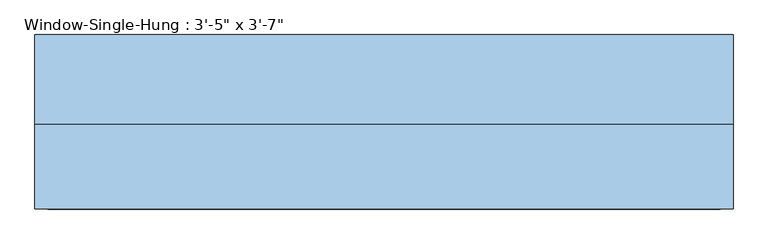
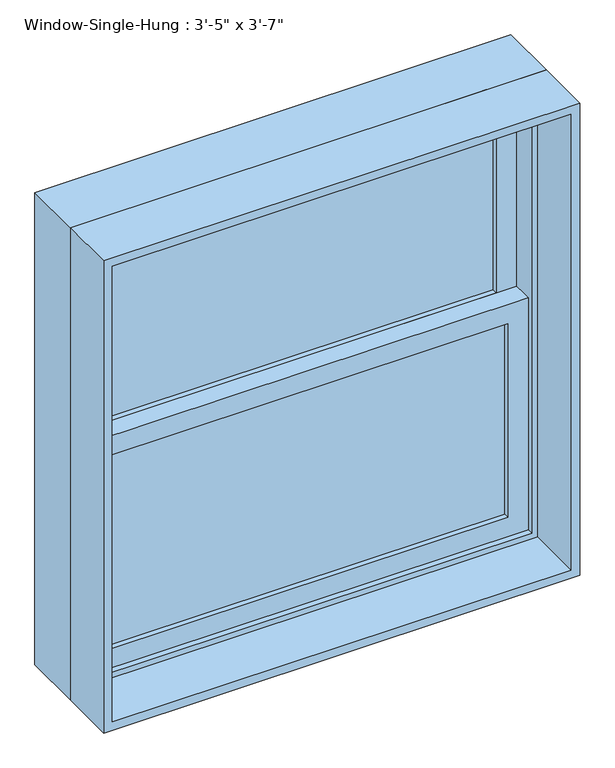
"""IFC4 building model written with IfcOpenShell, lengths in millimetres: window geometry."""

import ifcopenshell
import ifcopenshell.guid

model = None  # the IFC model being written
_history = None  # IfcOwnerHistory: only IFC2X3 demands one
_inside = {}  # id of a spatial element -> (the spatial element, [elements in it])
_under = {}  # id of a project, library or spatial element -> (it, [spatial elements below it])
_declared = {}  # id of a project -> (the project, [libraries it declares])
_typed = {}  # id of a type object -> (the type object, [elements of that type])
_made_of = {}  # id of a material, layer set ... -> (it, [elements and type objects made of it])


def new_model(schema):
    """Start an empty IFC model of exactly this schema.

    Asked for "IFC4X3", IfcOpenShell would pick the latest addendum, in which some entities
    have other attributes; the version numbers below select the first issue.
    IFC2X3 requires an IfcOwnerHistory on every rooted entity: one is made here for all.
    """
    global model, _history
    if schema == "IFC4X3":
        model = ifcopenshell.file(schema_version=(4, 3, 0, 0))
    else:
        model = ifcopenshell.file(schema=schema)
    _inside.clear()
    _under.clear()
    _declared.clear()
    _typed.clear()
    _made_of.clear()
    _history = None
    if model.schema == "IFC2X3":
        org = make("IfcOrganization", Name="unknown")
        user = make(
            "IfcPersonAndOrganization",
            ThePerson=make("IfcPerson", FamilyName="unknown"),
            TheOrganization=org,
        )
        app = make(
            "IfcApplication",
            ApplicationDeveloper=org,
            Version="unknown",
            ApplicationFullName="unknown",
            ApplicationIdentifier="unknown",
        )
        _history = make(
            "IfcOwnerHistory",
            OwningUser=user,
            OwningApplication=app,
            ChangeAction="ADDED",
            CreationDate=0,
        )
    return model


def make(cls, **values):
    """One entity of the class cls with the attributes given. An attribute that is None is left unset."""
    return model.create_entity(
        cls, **{name: value for name, value in values.items() if value is not None}
    )


def rooted(cls, **values):
    """An entity with a GlobalId (a new one), such as an element, a storey or a relation."""
    return make(cls, GlobalId=ifcopenshell.guid.new(), OwnerHistory=_history, **values)


def si_unit(unit_type, name, prefix=None):
    """IfcSIUnit, for example si_unit("LENGTHUNIT", "METRE", prefix="MILLI")."""
    return make("IfcSIUnit", UnitType=unit_type, Prefix=prefix, Name=name)


def assignment(units):
    """IfcUnitAssignment: the units of a project."""
    return None if units is None else make("IfcUnitAssignment", Units=units)


def point(xyz):
    """IfcCartesianPoint."""
    return None if xyz is None else make("IfcCartesianPoint", Coordinates=xyz)


def direction(xyz):
    """IfcDirection."""
    return None if xyz is None else make("IfcDirection", DirectionRatios=xyz)


def frame(location, z_axis=None, x_axis=None):
    """IfcAxis2Placement3D, a coordinate frame: its origin and axes. An axis left out is left unset."""
    return make(
        "IfcAxis2Placement3D",
        Location=point(location),
        Axis=direction(z_axis),
        RefDirection=direction(x_axis),
    )


def origin():
    """The frame at (0, 0, 0) with its axes left unset."""
    return frame((0.0, 0.0, 0.0))


def place(relative_to, where):
    """IfcLocalPlacement: puts the frame where relative to a parent placement (None: the world)."""
    return make(
        "IfcLocalPlacement", PlacementRelTo=relative_to, RelativePlacement=where
    )


def context(
    kind, dimensions, precision=None, world=None, true_north=None, identifier=None
):
    """IfcGeometricRepresentationContext, for example the 3D "Model" context."""
    return make(
        "IfcGeometricRepresentationContext",
        ContextIdentifier=identifier,
        ContextType=kind,
        CoordinateSpaceDimension=dimensions,
        Precision=precision,
        WorldCoordinateSystem=world,
        TrueNorth=true_north,
    )


def project(units=None, contexts=None):
    """IfcProject with its units and contexts."""
    return rooted(
        "IfcProject",
        Name="project",
        RepresentationContexts=contexts,
        UnitsInContext=assignment(units),
    )


def spatial(cls, under=None, at=None, **own):
    """A site, building, storey or space (cls), placed at a placement, below another one or the project."""
    s = rooted(cls, ObjectPlacement=at, **own)
    if under is not None:
        _under.setdefault(under.id(), (under, []))[1].append(s)
    return s


def polyline(points):
    """IfcPolyline through the points."""
    return make("IfcPolyline", Points=[point(p) for p in points])


def outline(outer, holes=None, kind="AREA"):
    """IfcArbitraryClosedProfileDef: a profile drawn as a closed curve; with holes, ...WithVoids."""
    if holes is None:
        return make("IfcArbitraryClosedProfileDef", ProfileType=kind, OuterCurve=outer)
    return make(
        "IfcArbitraryProfileDefWithVoids",
        ProfileType=kind,
        OuterCurve=outer,
        InnerCurves=holes,
    )


def extrude(swept, where, along, depth):
    """IfcExtrudedAreaSolid: the profile swept, set in the frame where, extruded along a direction by depth."""
    return make(
        "IfcExtrudedAreaSolid",
        SweptArea=swept,
        Position=where,
        ExtrudedDirection=direction(along),
        Depth=depth,
    )


def shape(context_of_items, identifier, shape_type, items):
    """IfcShapeRepresentation: the items that make up one representation, for example the "Body"."""
    return make(
        "IfcShapeRepresentation",
        ContextOfItems=context_of_items,
        RepresentationIdentifier=identifier,
        RepresentationType=shape_type,
        Items=items,
    )


def source(mapping_origin, context_of_items, identifier, shape_type, items):
    """IfcRepresentationMap: a shape defined once, which mapped items show again and again."""
    return make(
        "IfcRepresentationMap",
        MappingOrigin=mapping_origin,
        MappedRepresentation=shape(context_of_items, identifier, shape_type, items),
    )


def transform(
    local_origin,
    x_axis=None,
    y_axis=None,
    z_axis=None,
    scale=None,
    scale2=None,
    scale3=None,
    uniform=True,
):
    """IfcCartesianTransformationOperator3D, or its non-uniform kind. x_axis, y_axis, z_axis: its Axis1, 2, 3."""
    if uniform:
        return make(
            "IfcCartesianTransformationOperator3D",
            Axis1=direction(x_axis),
            Axis2=direction(y_axis),
            LocalOrigin=point(local_origin),
            Scale=scale,
            Axis3=direction(z_axis),
        )
    return make(
        "IfcCartesianTransformationOperator3DnonUniform",
        Axis1=direction(x_axis),
        Axis2=direction(y_axis),
        LocalOrigin=point(local_origin),
        Scale=scale,
        Axis3=direction(z_axis),
        Scale2=scale2,
        Scale3=scale3,
    )


def mapped(mapping_source, mapping_target):
    """IfcMappedItem: shows the shape of a source again, moved by a transform."""
    return make(
        "IfcMappedItem", MappingSource=mapping_source, MappingTarget=mapping_target
    )


def made_of(thing, what):
    """Note that an element or type object is made of a material, layer set ...; save() writes the relation."""
    if what is not None:
        _made_of.setdefault(what.id(), (what, []))[1].append(thing)
    return thing


def element(
    cls,
    number,
    at=None,
    inside=None,
    cuts=None,
    type_object=None,
    material=None,
    context=None,
    identifier="Body",
    shape_type=None,
    held_by="IfcProductDefinitionShape",
    body=None,
    shapes=None,
    **own,
):
    """One element of the class cls, such as IfcWall. Its Tag is "e" and its number.

    at: its placement. inside: the storey or other place that contains it. cuts: it is an
    opening in that element (IfcRelVoidsElement). A single representation is given by context,
    identifier, shape_type and body (its items); several are given by shapes. held_by: the class
    of the entity that holds the representations. save() writes the other relations.
    """
    e = rooted(cls, Tag="e%d" % number, ObjectPlacement=at, **own)
    if body is not None:
        shapes = [shape(context, identifier, shape_type, body)]
    if shapes is not None:
        e.Representation = make(held_by, Representations=shapes)
    if inside is not None:
        _inside.setdefault(inside.id(), (inside, []))[1].append(e)
    if cuts is not None:
        rooted(
            "IfcRelVoidsElement", RelatingBuildingElement=cuts, RelatedOpeningElement=e
        )
    if type_object is not None:
        _typed.setdefault(type_object.id(), (type_object, []))[1].append(e)
    return made_of(e, material)


def aggregate(whole, parts):
    """IfcRelAggregates: a whole, such as a stair, and the parts it consists of."""
    return rooted("IfcRelAggregates", RelatingObject=whole, RelatedObjects=parts)


def save(model, path):
    """Write the relations noted so far, then the file.

    IfcRelAggregates (storeys below a building ...), IfcRelContainedInSpatialStructure (elements
    in a storey), IfcRelDefinesByType, IfcRelAssociatesMaterial and IfcRelDeclares: one each for
    every whole, place, type object, material and project.
    """
    for whole, parts in _under.values():
        aggregate(whole, parts)
    for where, things in _inside.values():
        rooted(
            "IfcRelContainedInSpatialStructure",
            RelatedElements=things,
            RelatingStructure=where,
        )
    for kind, things in _typed.values():
        rooted("IfcRelDefinesByType", RelatedObjects=things, RelatingType=kind)
    for what, things in _made_of.values():
        rooted("IfcRelAssociatesMaterial", RelatedObjects=things, RelatingMaterial=what)
    for by, libraries in _declared.values():
        rooted("IfcRelDeclares", RelatingContext=by, RelatedDefinitions=libraries)
    model.write(path)


def window_d175fa0a(model_context):
    return source(origin(), model_context, "Body", "SweptSolid", [
        extrude(outline(polyline([(444.5, 50.8), (444.5, 44.45), (-444.5, 44.45), (-444.5, 50.8), (444.5, 50.8)])), frame((0.0, 0.0, 990.6), z_axis=(0.0, 0.0, 1.0), x_axis=(1.0, 0.0, 0.0)), (0.0, 0.0, 1.0), 447.675),
        extrude(outline(polyline([(-444.5, 38.1), (444.5, 38.1), (444.5, 31.75), (-444.5, 31.75), (-444.5, 38.1)])), frame((0.0, 0.0, 990.6), z_axis=(0.0, 0.0, 1.0), x_axis=(1.0, 0.0, 0.0)), (0.0, 0.0, 1.0), 447.675),
        extrude(outline(polyline([(444.5, 95.25), (444.5, 88.9), (-444.5, 88.9), (-444.5, 95.25), (444.5, 95.25)])), frame((0.0, 0.0, 1482.725), z_axis=(0.0, 0.0, 1.0), x_axis=(1.0, 0.0, 0.0)), (0.0, 0.0, 1.0), 447.675),
        extrude(outline(polyline([(-444.5, 82.55), (444.5, 82.55), (444.5, 76.2), (-444.5, 76.2), (-444.5, 82.55)])), frame((0.0, 0.0, 1482.725), z_axis=(0.0, 0.0, 1.0), x_axis=(1.0, 0.0, 0.0)), (0.0, 0.0, 1.0), 447.675),
        extrude(outline(polyline([(1482.725, -488.95), (946.15, -488.95), (946.15, 488.95), (1482.725, 488.95), (1482.725, -488.95)]), holes=[polyline([(1438.275, 444.5), (990.6, 444.5), (990.6, -444.5), (1438.275, -444.5), (1438.275, 444.5)])]), frame((0.0, 19.05, 0.0), z_axis=(0.0, 1.0, 0.0), x_axis=(0.0, 0.0, 1.0)), (0.0, 0.0, 1.0), 44.45),
        extrude(outline(polyline([(1974.85, -488.95), (1438.275, -488.95), (1438.275, 488.95), (1974.85, 488.95), (1974.85, -488.95)]), holes=[polyline([(1930.4, 444.5), (1482.725, 444.5), (1482.725, -444.5), (1930.4, -444.5), (1930.4, 444.5)])]), frame((0.0, 63.5, 0.0), z_axis=(0.0, 1.0, 0.0), x_axis=(0.0, 0.0, 1.0)), (0.0, 0.0, 1.0), 44.45),
        extrude(outline(polyline([(2006.6, -520.7), (914.4, -520.7), (914.4, 520.7), (2006.6, 520.7), (2006.6, -520.7)]), holes=[polyline([(1974.85, 488.95), (946.15, 488.95), (946.15, -488.95), (1974.85, -488.95), (1974.85, 488.95)])]), frame((0.0, 6.35, 0.0), z_axis=(0.0, 1.0, 0.0), x_axis=(0.0, 0.0, 1.0)), (0.0, 0.0, 1.0), 133.35),
        extrude(outline(polyline([(2006.6, 520.7), (2006.6, -520.7), (914.4, -520.7), (914.4, 520.7), (2006.6, 520.7)]), holes=[polyline([(1987.55, 501.65), (933.45, 501.65), (933.45, -501.65), (1987.55, -501.65), (1987.55, 501.65)])]), frame((0.0, -120.65, 0.0), z_axis=(0.0, 1.0, 0.0), x_axis=(0.0, 0.0, 1.0)), (0.0, 0.0, 1.0), 127.0),
    ])


if __name__ == "__main__":
    model = new_model("IFC4")
    model_context = context("Model", 3, world=origin())
    ifc_project = project(units=[si_unit("LENGTHUNIT", "METRE", prefix="MILLI")], contexts=[model_context])
    site = spatial("IfcSite", under=ifc_project)
    building = spatial("IfcBuilding", under=site)
    placement = place(None, origin())
    window_shape = window_d175fa0a(model_context)
    element("IfcWindow", 1, ObjectType="Window-Single-Hung : 3'-5\" x 3'-7\"", at=placement, inside=building, context=model_context, shape_type="MappedRepresentation", body=[
        mapped(window_shape, transform((0.0, 0.0, 0.0), x_axis=(1.0, 0.0, 0.0), y_axis=(0.0, 1.0, 0.0), z_axis=(0.0, 0.0, 1.0))),
    ])
    save(model, "model.ifc")

# Revit data of these elements
# Type "Window-Single-Hung : 3'-5\" x 3'-7\""
#   Type Mark = "25"
#   Fire Rating = "0.5h"
#   Construction Type Id = "DG-DR"
#   Assembly Code = "B2020100"
#   Analytic Construction = "Double glazing - domestic"
#   Wall Thickness [instance default] = 0' - 6"
#   Window Inset [instance default] = 0' - 0"
#   Visual Light Transmittance = 0.81
#   Thermal Resistance (R) = 0.319569 (m²·K)/W
#   Solar Heat Gain Coefficient = 0.76
#   Muntin Width = 2' - 11"
#   Muntin Height = 1' - 5 5/8"
#   Interior Wall Closure [instance default] = 0' - 1 1/2"
#   Rough Width = 3' - 5 1/2"
#   Rough Height = 3' - 7 1/2"
#   Frame Extension [instance default] = 0' - 1 1/4"
#   Exterior Wall Closure [instance default] = 0' - 0 1/2"
#   Extension Jamb [instance default] = 0' - 1 1/2"
#   Heat Transfer Coefficient (U) = 3.12929 W/(m²·K)
#   Height = 3' - 7"
#   Width = 3' - 5"
#   Top Muntin Visibility = no
#   Indicator Visibility = no
#   Extension Jamb Visibility [instance default] = yes
#   Interior Trim Visibility [instance default] = yes
#   Exterior Trim Visibility [instance default] = yes
#   Bottom Muntin Visibility = no
#   Muntin Pattern = Muntin Pattern_2x2 : Muntin Pattern_2x2
#   Interior Trim Material = Wood - Stained
#   Interior Trim = Trim-Window-Interior-Flat : Picture Frame
#   Exterior Trim Material = Clad - White
#   Exterior Trim = Trim-Window-Exterior-Flat : with Sill
#   Glass Panel Material = Glass
#   Exterior Frame Material = Clad - White
#   Interior Frame Material = Wood - Stained
#   Wall Closure = (empty or 0)
# Element 1 (IfcWindow, "Window-Single-Hung : 3'-5\" x 3'-7\"")
#   Wall Thickness = 0' - 9 1/2"
#   Extension Jamb = 0' - 5"
#   Materials on its faces: "Wood - Stained", "Glass", "Clad - White"
# Materials
#   "Wood - Stained": class "Wood", colour RGB 224 178 126, transparency 0, Cost = 0
#   "Clad - White": class "Wood", colour RGB 242 242 238, transparency 0, Cost = 0
#   "Glass": class "Glass", colour RGB 218 227 224, transparency 0.85, Description = "Soda Lime Glass", Cost = 0
